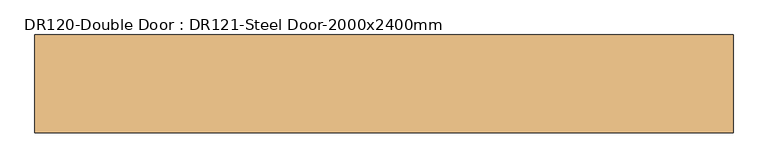
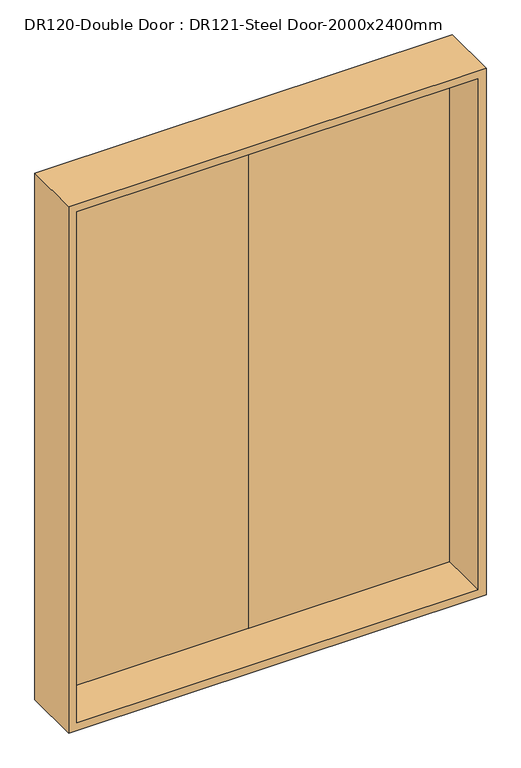
"""IFC4 building model written with IfcOpenShell, lengths in millimetres: door geometry, DR120-Double Door : DR121-Steel Door-2000x2400mm."""

from ifc_helpers import new_model, si_unit, frame, origin, place, context, project, spatial, polyline, outline, extrude, faceted_brep, source, transform, mapped, element, save


def dr120_double_door_dr121_steel_door_2000x2400mm_712166db(model_context):
    return source(origin(), model_context, "Body", "SolidModel", [
        extrude(outline(polyline([(880.0, 86.0), (0.0, 86.0), (0.0, 126.0), (880.0, 126.0), (880.0, 86.0)])), frame((0.0, 0.0, 20.0), z_axis=(0.0, 0.0, 1.0), x_axis=(1.0, 0.0, 0.0)), (0.0, 0.0, 1.0), 2360.0),
        extrude(outline(polyline([(0.0, 86.0), (-880.0, 86.0), (-880.0, 126.0), (0.0, 126.0), (0.0, 86.0)])), frame((0.0, 0.0, 20.0), z_axis=(0.0, 0.0, 1.0), x_axis=(1.0, 0.0, 0.0)), (0.0, 0.0, 1.0), 2360.0),
        faceted_brep([(900.0, -126.0, 2400.0), (900.0, 126.0, 2400.0), (-900.0, 126.0, 2400.0), (-900.0, -126.0, 2400.0), (865.0, 86.0, 2365.0), (865.0, -126.0, 2365.0), (-865.0, -126.0, 2365.0), (-865.0, 86.0, 2365.0), (880.0, 126.0, 2380.0), (880.0, 86.0, 2380.0), (-880.0, 86.0, 2380.0), (-880.0, 126.0, 2380.0), (-900.0, 126.0, 0.0), (-900.0, -126.0, 0.0), (-865.0, -126.0, 35.0), (-865.0, 86.0, 35.0), (-880.0, 86.0, 20.0), (-880.0, 126.0, 20.0), (900.0, 126.0, 0.0), (880.0, 126.0, 20.0), (900.0, -126.0, 0.0), (865.0, -126.0, 35.0), (865.0, 86.0, 35.0), (880.0, 86.0, 20.0)], [[[0, 1, 2, 3]], [[4, 5, 6, 7]], [[8, 9, 10, 11]], [[3, 2, 12, 13]], [[7, 6, 14, 15]], [[11, 10, 16, 17]], [[18, 12, 2, 1], [8, 11, 17, 19]], [[13, 12, 18, 20]], [[0, 3, 13, 20], [21, 14, 6, 5]], [[15, 14, 21, 22]], [[23, 16, 10, 9], [4, 7, 15, 22]], [[17, 16, 23, 19]], [[20, 18, 1, 0]], [[22, 21, 5, 4]], [[19, 23, 9, 8]]]),
    ])


if __name__ == "__main__":
    model = new_model("IFC4")
    model_context = context("Model", 3, world=origin())
    ifc_project = project(units=[si_unit("LENGTHUNIT", "METRE", prefix="MILLI")], contexts=[model_context])
    site = spatial("IfcSite", under=ifc_project)
    building = spatial("IfcBuilding", under=site)
    placement = place(None, origin())
    dr120_double_door_dr121_steel_door_2000x2400mm_shape = dr120_double_door_dr121_steel_door_2000x2400mm_712166db(model_context)
    element("IfcDoor", 1, ObjectType="DR120-Double Door : DR121-Steel Door-2000x2400mm", at=placement, inside=building, context=model_context, shape_type="MappedRepresentation", body=[
        mapped(dr120_double_door_dr121_steel_door_2000x2400mm_shape, transform((0.0, 0.0, 0.0), x_axis=(1.0, 0.0, 0.0), y_axis=(0.0, 1.0, 0.0), z_axis=(0.0, 0.0, 1.0))),
    ])
    save(model, "model.ifc")

# Revit data of these elements
# Type "DR120-Double Door : DR121-Steel Door-2000x2400mm"
#   Type Mark = "SD"
#   프레임 = ""
#   철물 = ""
#   유리/마감 = ""
#   위치/개소 = ""
#   부호 = "1/SD"
#   문번호 = ""
#   문기호 = "SD"
#   Analytic Construction = "<None>"
#   Height = 2400 mm
#   Width = 1800 mm
#   Define Thermal Properties by = 1
#   문 틀 = A04AQ098-00003_Steel Door_non FP_double
#   문 = 문
#   Function = (empty or 0)
#   Assembly Code = ""
#   Wall Closure = (empty or 0)
# Element 1 (IfcDoor, "DR120-Double Door : DR121-Steel Door-2000x2400mm")
#   Materials on its faces: "A04AQ098-00003_Steel Door_non FP_double", "문"
# Materials
#   "A04AQ098-00003_Steel Door_non FP_double": class "금속", colour RGB 247 247 247, transparency 0, Description = "Steel Door", W00) Work Master Code = "A04AQ098-00003", W01) Work Master_Lv1 = "Finishing Work", W02) Work Master_Lv2 = "Door & Window Work", W03) Work Master_Spec.1 = "Steel Door w/ Steel Frame", W04) Work Master_Spec.2 = "Fire Protective Rating: N/A, Double Door", W05) Work Master_Spec.3 = "w/ Hardware & Accessories", Cost = 0
#   "문": class "다양한", colour RGB 247 247 247, transparency 0
